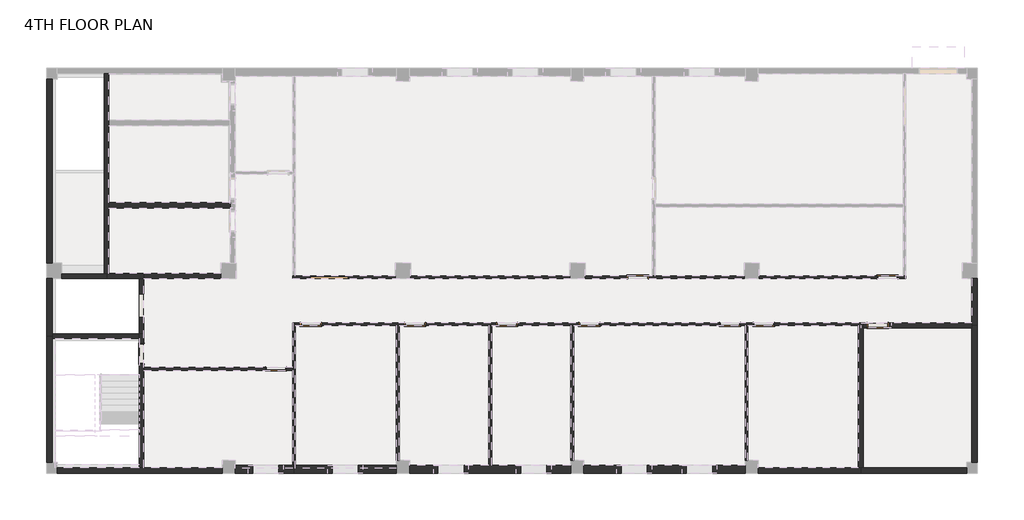
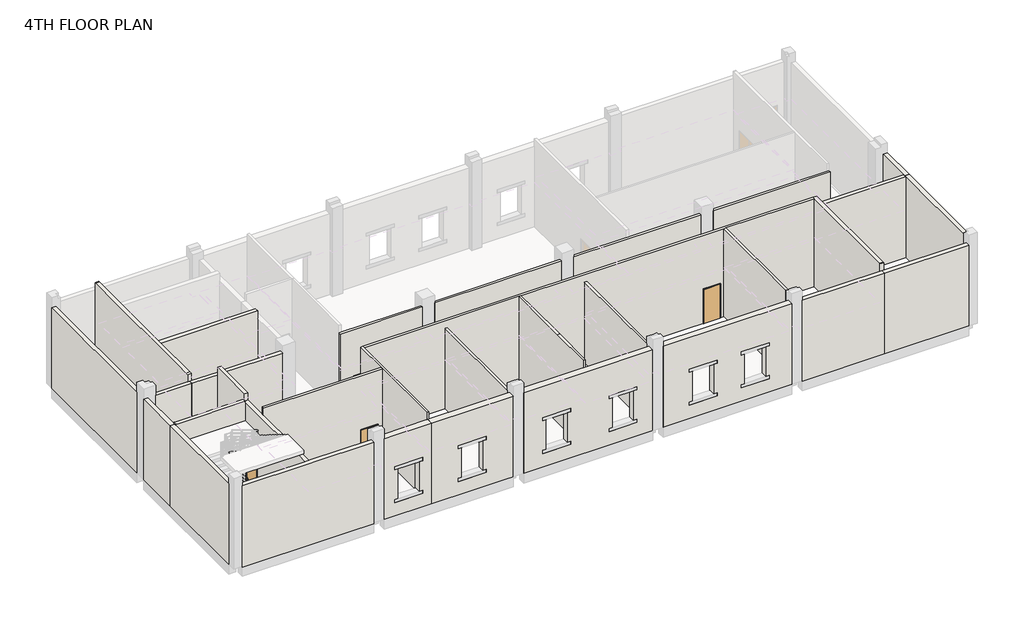
# One storey, part 1 of 6: 34 walls, 12 doors.
"""IFC4 building model written with IfcOpenShell, lengths in millimetres."""

import ifcopenshell
import ifcopenshell.guid

model = None  # the IFC model being written
_history = None  # IfcOwnerHistory: only IFC2X3 demands one
_inside = {}  # id of a spatial element -> (the spatial element, [elements in it])
_under = {}  # id of a project, library or spatial element -> (it, [spatial elements below it])
_declared = {}  # id of a project -> (the project, [libraries it declares])
_typed = {}  # id of a type object -> (the type object, [elements of that type])
_made_of = {}  # id of a material, layer set ... -> (it, [elements and type objects made of it])


def new_model(schema):
    """Start an empty IFC model of exactly this schema.

    Asked for "IFC4X3", IfcOpenShell would pick the latest addendum, in which some entities
    have other attributes; the version numbers below select the first issue.
    IFC2X3 requires an IfcOwnerHistory on every rooted entity: one is made here for all.
    """
    global model, _history
    if schema == "IFC4X3":
        model = ifcopenshell.file(schema_version=(4, 3, 0, 0))
    else:
        model = ifcopenshell.file(schema=schema)
    _inside.clear()
    _under.clear()
    _declared.clear()
    _typed.clear()
    _made_of.clear()
    _history = None
    if model.schema == "IFC2X3":
        org = make("IfcOrganization", Name="unknown")
        user = make(
            "IfcPersonAndOrganization",
            ThePerson=make("IfcPerson", FamilyName="unknown"),
            TheOrganization=org,
        )
        app = make(
            "IfcApplication",
            ApplicationDeveloper=org,
            Version="unknown",
            ApplicationFullName="unknown",
            ApplicationIdentifier="unknown",
        )
        _history = make(
            "IfcOwnerHistory",
            OwningUser=user,
            OwningApplication=app,
            ChangeAction="ADDED",
            CreationDate=0,
        )
    return model


def make(cls, **values):
    """One entity of the class cls with the attributes given. An attribute that is None is left unset."""
    return model.create_entity(
        cls, **{name: value for name, value in values.items() if value is not None}
    )


def rooted(cls, **values):
    """An entity with a GlobalId (a new one), such as an element, a storey or a relation."""
    return make(cls, GlobalId=ifcopenshell.guid.new(), OwnerHistory=_history, **values)


def si_unit(unit_type, name, prefix=None):
    """IfcSIUnit, for example si_unit("LENGTHUNIT", "METRE", prefix="MILLI")."""
    return make("IfcSIUnit", UnitType=unit_type, Prefix=prefix, Name=name)


def assignment(units):
    """IfcUnitAssignment: the units of a project."""
    return None if units is None else make("IfcUnitAssignment", Units=units)


def point(xyz):
    """IfcCartesianPoint."""
    return None if xyz is None else make("IfcCartesianPoint", Coordinates=xyz)


def direction(xyz):
    """IfcDirection."""
    return None if xyz is None else make("IfcDirection", DirectionRatios=xyz)


def frame(location, z_axis=None, x_axis=None):
    """IfcAxis2Placement3D, a coordinate frame: its origin and axes. An axis left out is left unset."""
    return make(
        "IfcAxis2Placement3D",
        Location=point(location),
        Axis=direction(z_axis),
        RefDirection=direction(x_axis),
    )


def origin():
    """The frame at (0, 0, 0) with its axes left unset."""
    return frame((0.0, 0.0, 0.0))


def origin_with_axes():
    """The frame at (0, 0, 0) with the z axis (0, 0, 1) and the x axis (1, 0, 0) written out."""
    return frame((0.0, 0.0, 0.0), z_axis=(0.0, 0.0, 1.0), x_axis=(1.0, 0.0, 0.0))


def place(relative_to, where):
    """IfcLocalPlacement: puts the frame where relative to a parent placement (None: the world)."""
    return make(
        "IfcLocalPlacement", PlacementRelTo=relative_to, RelativePlacement=where
    )


def context(
    kind, dimensions, precision=None, world=None, true_north=None, identifier=None
):
    """IfcGeometricRepresentationContext, for example the 3D "Model" context."""
    return make(
        "IfcGeometricRepresentationContext",
        ContextIdentifier=identifier,
        ContextType=kind,
        CoordinateSpaceDimension=dimensions,
        Precision=precision,
        WorldCoordinateSystem=world,
        TrueNorth=true_north,
    )


def project(units=None, contexts=None):
    """IfcProject with its units and contexts."""
    return rooted(
        "IfcProject",
        Name="project",
        RepresentationContexts=contexts,
        UnitsInContext=assignment(units),
    )


def spatial(cls, under=None, at=None, **own):
    """A site, building, storey or space (cls), placed at a placement, below another one or the project."""
    s = rooted(cls, ObjectPlacement=at, **own)
    if under is not None:
        _under.setdefault(under.id(), (under, []))[1].append(s)
    return s


def polyline(points):
    """IfcPolyline through the points."""
    return make("IfcPolyline", Points=[point(p) for p in points])


def outline(outer, holes=None, kind="AREA"):
    """IfcArbitraryClosedProfileDef: a profile drawn as a closed curve; with holes, ...WithVoids."""
    if holes is None:
        return make("IfcArbitraryClosedProfileDef", ProfileType=kind, OuterCurve=outer)
    return make(
        "IfcArbitraryProfileDefWithVoids",
        ProfileType=kind,
        OuterCurve=outer,
        InnerCurves=holes,
    )


def extrude(swept, where, along, depth):
    """IfcExtrudedAreaSolid: the profile swept, set in the frame where, extruded along a direction by depth."""
    return make(
        "IfcExtrudedAreaSolid",
        SweptArea=swept,
        Position=where,
        ExtrudedDirection=direction(along),
        Depth=depth,
    )


def faces_of(points, faces, orient=None, outer=None):
    """IfcFace entities. A face is a list of loops; a loop is a list of indices into points, from 0.

    orient and outer hold one flag for each loop. By default every Orientation is true, the
    first loop of a face is its IfcFaceOuterBound and the others are IfcFaceBound.
    """
    made = []
    for i, loops in enumerate(faces):
        bounds = []
        for j, loop in enumerate(loops):
            is_outer = j == 0 if outer is None else outer[i][j]
            bounds.append(
                make(
                    "IfcFaceOuterBound" if is_outer else "IfcFaceBound",
                    Bound=make("IfcPolyLoop", Polygon=[points[k] for k in loop]),
                    Orientation=True if orient is None else orient[i][j],
                )
            )
        made.append(make("IfcFace", Bounds=bounds))
    return made


def faceted_brep(points, faces, orient=None, outer=None, voids=None):
    """IfcFacetedBrep: a solid bounded by flat faces; with voids (closed shells), ...WithVoids."""
    shared = [point(p) for p in points]
    hull = make("IfcClosedShell", CfsFaces=faces_of(shared, faces, orient, outer))
    if voids is None:
        return make("IfcFacetedBrep", Outer=hull)
    return make(
        "IfcFacetedBrepWithVoids",
        Outer=hull,
        Voids=[
            make(cls, CfsFaces=faces_of(shared, fs, o, b)) for cls, fs, o, b in voids
        ],
    )


def shape(context_of_items, identifier, shape_type, items):
    """IfcShapeRepresentation: the items that make up one representation, for example the "Body"."""
    return make(
        "IfcShapeRepresentation",
        ContextOfItems=context_of_items,
        RepresentationIdentifier=identifier,
        RepresentationType=shape_type,
        Items=items,
    )


def source(mapping_origin, context_of_items, identifier, shape_type, items):
    """IfcRepresentationMap: a shape defined once, which mapped items show again and again."""
    return make(
        "IfcRepresentationMap",
        MappingOrigin=mapping_origin,
        MappedRepresentation=shape(context_of_items, identifier, shape_type, items),
    )


def transform(
    local_origin,
    x_axis=None,
    y_axis=None,
    z_axis=None,
    scale=None,
    scale2=None,
    scale3=None,
    uniform=True,
):
    """IfcCartesianTransformationOperator3D, or its non-uniform kind. x_axis, y_axis, z_axis: its Axis1, 2, 3."""
    if uniform:
        return make(
            "IfcCartesianTransformationOperator3D",
            Axis1=direction(x_axis),
            Axis2=direction(y_axis),
            LocalOrigin=point(local_origin),
            Scale=scale,
            Axis3=direction(z_axis),
        )
    return make(
        "IfcCartesianTransformationOperator3DnonUniform",
        Axis1=direction(x_axis),
        Axis2=direction(y_axis),
        LocalOrigin=point(local_origin),
        Scale=scale,
        Axis3=direction(z_axis),
        Scale2=scale2,
        Scale3=scale3,
    )


def mapped(mapping_source, mapping_target):
    """IfcMappedItem: shows the shape of a source again, moved by a transform."""
    return make(
        "IfcMappedItem", MappingSource=mapping_source, MappingTarget=mapping_target
    )


def made_of(thing, what):
    """Note that an element or type object is made of a material, layer set ...; save() writes the relation."""
    if what is not None:
        _made_of.setdefault(what.id(), (what, []))[1].append(thing)
    return thing


def element(
    cls,
    number,
    at=None,
    inside=None,
    cuts=None,
    type_object=None,
    material=None,
    context=None,
    identifier="Body",
    shape_type=None,
    held_by="IfcProductDefinitionShape",
    body=None,
    shapes=None,
    **own,
):
    """One element of the class cls, such as IfcWall. Its Tag is "e" and its number.

    at: its placement. inside: the storey or other place that contains it. cuts: it is an
    opening in that element (IfcRelVoidsElement). A single representation is given by context,
    identifier, shape_type and body (its items); several are given by shapes. held_by: the class
    of the entity that holds the representations. save() writes the other relations.
    """
    e = rooted(cls, Tag="e%d" % number, ObjectPlacement=at, **own)
    if body is not None:
        shapes = [shape(context, identifier, shape_type, body)]
    if shapes is not None:
        e.Representation = make(held_by, Representations=shapes)
    if inside is not None:
        _inside.setdefault(inside.id(), (inside, []))[1].append(e)
    if cuts is not None:
        rooted(
            "IfcRelVoidsElement", RelatingBuildingElement=cuts, RelatedOpeningElement=e
        )
    if type_object is not None:
        _typed.setdefault(type_object.id(), (type_object, []))[1].append(e)
    return made_of(e, material)


def aggregate(whole, parts):
    """IfcRelAggregates: a whole, such as a stair, and the parts it consists of."""
    return rooted("IfcRelAggregates", RelatingObject=whole, RelatedObjects=parts)


def save(model, path):
    """Write the relations noted so far, then the file.

    IfcRelAggregates (storeys below a building ...), IfcRelContainedInSpatialStructure (elements
    in a storey), IfcRelDefinesByType, IfcRelAssociatesMaterial and IfcRelDeclares: one each for
    every whole, place, type object, material and project.
    """
    for whole, parts in _under.values():
        aggregate(whole, parts)
    for where, things in _inside.values():
        rooted(
            "IfcRelContainedInSpatialStructure",
            RelatedElements=things,
            RelatingStructure=where,
        )
    for kind, things in _typed.values():
        rooted("IfcRelDefinesByType", RelatedObjects=things, RelatingType=kind)
    for what, things in _made_of.values():
        rooted("IfcRelAssociatesMaterial", RelatedObjects=things, RelatingMaterial=what)
    for by, libraries in _declared.values():
        rooted("IfcRelDeclares", RelatingContext=by, RelatedDefinitions=libraries)
    model.write(path)


def dr110_single_door_dr111_steel_door_1000x2100mm_481420e4(model_context):
    return source(origin(), model_context, "Body", "SolidModel", [
        extrude(outline(polyline([(470.0, -141.0), (-470.0, -141.0), (-470.0, -106.0), (470.0, -106.0), (470.0, -141.0)])), origin_with_axes(), (0.0, 0.0, 1.0), 2070.0),
        faceted_brep([(470.0, -141.0, 0.0), (470.0, -106.0, 0.0), (450.0, -106.0, 0.0), (450.0, 106.0, 0.0), (470.0, 106.0, 0.0), (470.0, 141.0, 0.0), (500.0, 141.0, 0.0), (500.0, -141.0, 0.0), (500.0, -141.0, 2100.0), (-500.0, -141.0, 2100.0), (-500.0, -141.0, 0.0), (-470.0, -141.0, 0.0), (-470.0, -141.0, 2070.0), (470.0, -141.0, 2070.0), (500.0, 141.0, 2100.0), (470.0, 141.0, 2070.0), (-470.0, 141.0, 2070.0), (-470.0, 141.0, 0.0), (-500.0, 141.0, 0.0), (-500.0, 141.0, 2100.0), (470.0, 106.0, 2070.0), (450.0, 106.0, 2050.0), (-450.0, 106.0, 2050.0), (-450.0, 106.0, 0.0), (-470.0, 106.0, 0.0), (-470.0, 106.0, 2070.0), (450.0, -106.0, 2050.0), (470.0, -106.0, 2070.0), (-470.0, -106.0, 2070.0), (-470.0, -106.0, 0.0), (-450.0, -106.0, 0.0), (-450.0, -106.0, 2050.0)], [[[0, 1, 2, 3, 4, 5, 6, 7]], [[7, 8, 9, 10, 11, 12, 13, 0]], [[6, 14, 8, 7]], [[5, 15, 16, 17, 18, 19, 14, 6]], [[4, 20, 15, 5]], [[3, 21, 22, 23, 24, 25, 20, 4]], [[2, 26, 21, 3]], [[1, 27, 28, 29, 30, 31, 26, 2]], [[0, 13, 27, 1]], [[12, 11, 29, 28]], [[11, 10, 18, 17, 24, 23, 30, 29]], [[19, 18, 10, 9]], [[25, 24, 17, 16]], [[31, 30, 23, 22]], [[14, 19, 9, 8]], [[20, 25, 16, 15]], [[26, 31, 22, 21]], [[13, 12, 28, 27]]]),
    ])


def dr110_single_door_dr111_steel_door_1000x2100mm_0699664c(model_context):
    return source(origin(), model_context, "Body", "SolidModel", [
        extrude(outline(polyline([(470.0, 92.5), (470.0, 57.5), (-470.0, 57.5), (-470.0, 92.5), (470.0, 92.5)])), origin_with_axes(), (0.0, 0.0, 1.0), 2070.0),
        faceted_brep([(470.0, 92.5, 0.0), (500.0, 92.5, 0.0), (500.0, -92.5, 0.0), (470.0, -92.5, 0.0), (470.0, -57.5, 0.0), (450.0, -57.5, 0.0), (450.0, 57.5, 0.0), (470.0, 57.5, 0.0), (470.0, 92.5, 2070.0), (-470.0, 92.5, 2070.0), (-470.0, 92.5, 0.0), (-500.0, 92.5, 0.0), (-500.0, 92.5, 2100.0), (500.0, 92.5, 2100.0), (500.0, -92.5, 2100.0), (-500.0, -92.5, 2100.0), (-500.0, -92.5, 0.0), (-470.0, -92.5, 0.0), (-470.0, -92.5, 2070.0), (470.0, -92.5, 2070.0), (470.0, -57.5, 2070.0), (-470.0, -57.5, 2070.0), (-470.0, -57.5, 0.0), (-450.0, -57.5, 0.0), (-450.0, -57.5, 2050.0), (450.0, -57.5, 2050.0), (450.0, 57.5, 2050.0), (-450.0, 57.5, 2050.0), (-450.0, 57.5, 0.0), (-470.0, 57.5, 0.0), (-470.0, 57.5, 2070.0), (470.0, 57.5, 2070.0)], [[[0, 1, 2, 3, 4, 5, 6, 7]], [[1, 0, 8, 9, 10, 11, 12, 13]], [[2, 1, 13, 14]], [[3, 2, 14, 15, 16, 17, 18, 19]], [[4, 3, 19, 20]], [[5, 4, 20, 21, 22, 23, 24, 25]], [[6, 5, 25, 26]], [[7, 6, 26, 27, 28, 29, 30, 31]], [[0, 7, 31, 8]], [[9, 30, 29, 10]], [[10, 29, 28, 23, 22, 17, 16, 11]], [[15, 12, 11, 16]], [[21, 18, 17, 22]], [[27, 24, 23, 28]], [[14, 13, 12, 15]], [[20, 19, 18, 21]], [[26, 25, 24, 27]], [[8, 31, 30, 9]]]),
    ])


def dr110_single_door_dr111_steel_door_1000x2100mm_67953bf6(model_context):
    return source(origin(), model_context, "Body", "SolidModel", [
        extrude(outline(polyline([(470.0, -92.5), (-470.0, -92.5), (-470.0, -57.5), (470.0, -57.5), (470.0, -92.5)])), origin_with_axes(), (0.0, 0.0, 1.0), 2070.0),
        faceted_brep([(470.0, -92.5, 0.0), (470.0, -57.5, 0.0), (450.0, -57.5, 0.0), (450.0, 57.5, 0.0), (470.0, 57.5, 0.0), (470.0, 92.5, 0.0), (500.0, 92.5, 0.0), (500.0, -92.5, 0.0), (500.0, -92.5, 2100.0), (-500.0, -92.5, 2100.0), (-500.0, -92.5, 0.0), (-470.0, -92.5, 0.0), (-470.0, -92.5, 2070.0), (470.0, -92.5, 2070.0), (500.0, 92.5, 2100.0), (470.0, 92.5, 2070.0), (-470.0, 92.5, 2070.0), (-470.0, 92.5, 0.0), (-500.0, 92.5, 0.0), (-500.0, 92.5, 2100.0), (470.0, 57.5, 2070.0), (450.0, 57.5, 2050.0), (-450.0, 57.5, 2050.0), (-450.0, 57.5, 0.0), (-470.0, 57.5, 0.0), (-470.0, 57.5, 2070.0), (450.0, -57.5, 2050.0), (470.0, -57.5, 2070.0), (-470.0, -57.5, 2070.0), (-470.0, -57.5, 0.0), (-450.0, -57.5, 0.0), (-450.0, -57.5, 2050.0)], [[[0, 1, 2, 3, 4, 5, 6, 7]], [[7, 8, 9, 10, 11, 12, 13, 0]], [[6, 14, 8, 7]], [[5, 15, 16, 17, 18, 19, 14, 6]], [[4, 20, 15, 5]], [[3, 21, 22, 23, 24, 25, 20, 4]], [[2, 26, 21, 3]], [[1, 27, 28, 29, 30, 31, 26, 2]], [[0, 13, 27, 1]], [[12, 11, 29, 28]], [[11, 10, 18, 17, 24, 23, 30, 29]], [[19, 18, 10, 9]], [[25, 24, 17, 16]], [[31, 30, 23, 22]], [[14, 19, 9, 8]], [[20, 25, 16, 15]], [[26, 31, 22, 21]], [[13, 12, 28, 27]]]),
    ])


def dr110_single_door_dr112_steel_door_1000x2100mm_panic_bar_81a01685(model_context):
    return source(origin(), model_context, "Body", "SolidModel", [
        extrude(outline(polyline([(470.0, -131.0), (-470.0, -131.0), (-470.0, -96.0), (470.0, -96.0), (470.0, -131.0)])), origin_with_axes(), (0.0, 0.0, 1.0), 2070.0),
        faceted_brep([(470.0, -131.0, 0.0), (470.0, -96.0, 0.0), (450.0, -96.0, 0.0), (450.0, 96.0, 0.0), (470.0, 96.0, 0.0), (470.0, 131.0, 0.0), (500.0, 131.0, 0.0), (500.0, -131.0, 0.0), (500.0, -131.0, 2100.0), (-500.0, -131.0, 2100.0), (-500.0, -131.0, 0.0), (-470.0, -131.0, 0.0), (-470.0, -131.0, 2070.0), (470.0, -131.0, 2070.0), (500.0, 131.0, 2100.0), (470.0, 131.0, 2070.0), (-470.0, 131.0, 2070.0), (-470.0, 131.0, 0.0), (-500.0, 131.0, 0.0), (-500.0, 131.0, 2100.0), (470.0, 96.0, 2070.0), (450.0, 96.0, 2050.0), (-450.0, 96.0, 2050.0), (-450.0, 96.0, 0.0), (-470.0, 96.0, 0.0), (-470.0, 96.0, 2070.0), (450.0, -96.0, 2050.0), (470.0, -96.0, 2070.0), (-470.0, -96.0, 2070.0), (-470.0, -96.0, 0.0), (-450.0, -96.0, 0.0), (-450.0, -96.0, 2050.0)], [[[0, 1, 2, 3, 4, 5, 6, 7]], [[7, 8, 9, 10, 11, 12, 13, 0]], [[6, 14, 8, 7]], [[5, 15, 16, 17, 18, 19, 14, 6]], [[4, 20, 15, 5]], [[3, 21, 22, 23, 24, 25, 20, 4]], [[2, 26, 21, 3]], [[1, 27, 28, 29, 30, 31, 26, 2]], [[0, 13, 27, 1]], [[12, 11, 29, 28]], [[11, 10, 18, 17, 24, 23, 30, 29]], [[19, 18, 10, 9]], [[25, 24, 17, 16]], [[31, 30, 23, 22]], [[14, 19, 9, 8]], [[20, 25, 16, 15]], [[26, 31, 22, 21]], [[13, 12, 28, 27]]]),
    ])


def dr120_double_door_dr121_steel_door_2000x2100mm_61964ec1(model_context):
    return source(origin(), model_context, "Body", "SolidModel", [
        extrude(outline(polyline([(880.0, 22.5), (0.0, 22.5), (0.0, 62.5), (880.0, 62.5), (880.0, 22.5)])), frame((0.0, 0.0, 20.0), z_axis=(0.0, 0.0, 1.0), x_axis=(1.0, 0.0, 0.0)), (0.0, 0.0, 1.0), 2060.0),
        extrude(outline(polyline([(0.0, 22.5), (-880.0, 22.5), (-880.0, 62.5), (0.0, 62.5), (0.0, 22.5)])), frame((0.0, 0.0, 20.0), z_axis=(0.0, 0.0, 1.0), x_axis=(1.0, 0.0, 0.0)), (0.0, 0.0, 1.0), 2060.0),
        faceted_brep([(900.0, -62.5, 2100.0), (900.0, 62.5, 2100.0), (-900.0, 62.5, 2100.0), (-900.0, -62.5, 2100.0), (865.0, 22.5, 2065.0), (865.0, -62.5, 2065.0), (-865.0, -62.5, 2065.0), (-865.0, 22.5, 2065.0), (880.0, 62.5, 2080.0), (880.0, 22.5, 2080.0), (-880.0, 22.5, 2080.0), (-880.0, 62.5, 2080.0), (-900.0, 62.5, 0.0), (-900.0, -62.5, 0.0), (-865.0, -62.5, 35.0), (-865.0, 22.5, 35.0), (-880.0, 22.5, 20.0), (-880.0, 62.5, 20.0), (900.0, 62.5, 0.0), (880.0, 62.5, 20.0), (900.0, -62.5, 0.0), (865.0, -62.5, 35.0), (865.0, 22.5, 35.0), (880.0, 22.5, 20.0)], [[[0, 1, 2, 3]], [[4, 5, 6, 7]], [[8, 9, 10, 11]], [[3, 2, 12, 13]], [[7, 6, 14, 15]], [[11, 10, 16, 17]], [[18, 12, 2, 1], [8, 11, 17, 19]], [[13, 12, 18, 20]], [[0, 3, 13, 20], [21, 14, 6, 5]], [[15, 14, 21, 22]], [[23, 16, 10, 9], [4, 7, 15, 22]], [[17, 16, 23, 19]], [[20, 18, 1, 0]], [[22, 21, 5, 4]], [[19, 23, 9, 8]]]),
    ])


model = new_model("IFC4")

# Units and contexts
model_context = context("Model", 3, world=origin())
ifc_project = project(units=[si_unit("LENGTHUNIT", "METRE", prefix="MILLI")], contexts=[model_context])

# Site, building, storey
site = spatial("IfcSite", under=ifc_project)
building = spatial("IfcBuilding", under=site)
storey = spatial("IfcBuildingStorey", under=building, Name="4TH FLOOR PLAN", Elevation=16100.005241)

# Doors
placement = place(None, origin())
dr110_single_door_dr111_steel_door_1000x2100mm_shape = dr110_single_door_dr111_steel_door_1000x2100mm_481420e4(model_context)
element("IfcDoor", 1, ObjectType="DR110-Single Door : DR111-Steel Door-1000x2100mm", at=placement, inside=storey, context=model_context, shape_type="MappedRepresentation", body=[
    mapped(dr110_single_door_dr111_steel_door_1000x2100mm_shape, transform((37775.0, 27499.5208589, 16100.005241), x_axis=(1.0, 0.0, 0.0), y_axis=(0.0, 1.0, 0.0), z_axis=(0.0, 0.0, 1.0))),
])
dr110_single_door_dr111_steel_door_1000x2100mm_2_shape = dr110_single_door_dr111_steel_door_1000x2100mm_0699664c(model_context)
element("IfcDoor", 2, ObjectType="DR110-Single Door : DR111-Steel Door-1000x2100mm", at=placement, inside=storey, context=model_context, shape_type="MappedRepresentation", body=[
    mapped(dr110_single_door_dr111_steel_door_1000x2100mm_2_shape, transform((10170.0, 25499.5208589, 16100.005241), x_axis=(-1.0, 0.0, 0.0), y_axis=(0.0, -1.0, 0.0), z_axis=(0.0, 0.0, 1.0))),
])
element("IfcDoor", 3, ObjectType="DR110-Single Door : DR111-Steel Door-1000x2100mm", at=placement, inside=storey, context=model_context, shape_type="MappedRepresentation", body=[
    mapped(dr110_single_door_dr111_steel_door_1000x2100mm_2_shape, transform((31000.0, 27547.0208589, 16100.005241), x_axis=(-1.0, 0.0, 0.0), y_axis=(0.0, -1.0, 0.0), z_axis=(0.0, 0.0, 1.0))),
])
dr110_single_door_dr111_steel_door_1000x2100mm_3_shape = dr110_single_door_dr111_steel_door_1000x2100mm_67953bf6(model_context)
element("IfcDoor", 4, ObjectType="DR110-Single Door : DR111-Steel Door-1000x2100mm", at=placement, inside=storey, context=model_context, shape_type="MappedRepresentation", body=[
    mapped(dr110_single_door_dr111_steel_door_1000x2100mm_3_shape, transform((38225.0, 29712.0208589, 16100.005241), x_axis=(-1.0, 0.0, 0.0), y_axis=(0.0, -1.0, 0.0), z_axis=(0.0, 0.0, 1.0))),
])
element("IfcDoor", 5, ObjectType="DR110-Single Door : DR111-Steel Door-1000x2100mm", at=placement, inside=storey, context=model_context, shape_type="MappedRepresentation", body=[
    mapped(dr110_single_door_dr111_steel_door_1000x2100mm_3_shape, transform((26770.0, 29712.0208589, 16100.005241), x_axis=(-1.0, 0.0, 0.0), y_axis=(0.0, -1.0, 0.0), z_axis=(0.0, 0.0, 1.0))),
])
element("IfcDoor", 6, ObjectType="DR110-Single Door : DR111-Steel Door-1000x2100mm", at=placement, inside=storey, context=model_context, shape_type="MappedRepresentation", body=[
    mapped(dr110_single_door_dr111_steel_door_1000x2100mm_3_shape, transform((11775.0, 27547.0208589, 16100.005241), x_axis=(1.0, 0.0, 0.0), y_axis=(0.0, 1.0, 0.0), z_axis=(0.0, 0.0, 1.0))),
])
element("IfcDoor", 7, ObjectType="DR110-Single Door : DR111-Steel Door-1000x2100mm", at=placement, inside=storey, context=model_context, shape_type="MappedRepresentation", body=[
    mapped(dr110_single_door_dr111_steel_door_1000x2100mm_3_shape, transform((16550.0, 27547.0208589, 16100.005241), x_axis=(1.0, 0.0, 0.0), y_axis=(0.0, 1.0, 0.0), z_axis=(0.0, 0.0, 1.0))),
])
element("IfcDoor", 8, ObjectType="DR110-Single Door : DR111-Steel Door-1000x2100mm", at=placement, inside=storey, context=model_context, shape_type="MappedRepresentation", body=[
    mapped(dr110_single_door_dr111_steel_door_1000x2100mm_3_shape, transform((20775.0, 27547.0208589, 16100.005241), x_axis=(1.0, 0.0, 0.0), y_axis=(0.0, 1.0, 0.0), z_axis=(0.0, 0.0, 1.0))),
])
element("IfcDoor", 9, ObjectType="DR110-Single Door : DR111-Steel Door-1000x2100mm", at=placement, inside=storey, context=model_context, shape_type="MappedRepresentation", body=[
    mapped(dr110_single_door_dr111_steel_door_1000x2100mm_3_shape, transform((24550.0, 27547.0208589, 16100.005241), x_axis=(1.0, 0.0, 0.0), y_axis=(0.0, 1.0, 0.0), z_axis=(0.0, 0.0, 1.0))),
])
element("IfcDoor", 10, ObjectType="DR110-Single Door : DR111-Steel Door-1000x2100mm", at=placement, inside=storey, context=model_context, shape_type="MappedRepresentation", body=[
    mapped(dr110_single_door_dr111_steel_door_1000x2100mm_3_shape, transform((32550.0, 27547.0208589, 16100.005241), x_axis=(1.0, 0.0, 0.0), y_axis=(0.0, 1.0, 0.0), z_axis=(0.0, 0.0, 1.0))),
])
dr110_single_door_dr112_steel_door_1000x2100mm_panic_bar_shape = dr110_single_door_dr112_steel_door_1000x2100mm_panic_bar_81a01685(model_context)
element("IfcDoor", 11, ObjectType="DR110-Single Door : DR112-Steel Door-1000x2100mm_Panic Bar", at=placement, inside=storey, context=model_context, shape_type="MappedRepresentation", body=[
    mapped(dr110_single_door_dr112_steel_door_1000x2100mm_panic_bar_shape, transform((4000.0, 26199.5208589, 16100.005241), x_axis=(0.0, -1.0, 0.0), y_axis=(1.0, 0.0, 0.0), z_axis=(0.0, 0.0, 1.0))),
])
dr120_double_door_dr121_steel_door_2000x2100mm_shape = dr120_double_door_dr121_steel_door_2000x2100mm_61964ec1(model_context)
element("IfcDoor", 12, ObjectType="DR120-Double Door : DR121-Steel Door-2000x2100mm", at=placement, inside=storey, context=model_context, shape_type="MappedRepresentation", body=[
    mapped(dr120_double_door_dr121_steel_door_2000x2100mm_shape, transform((12620.0, 29712.0208589, 16100.005241), x_axis=(1.0, 0.0, 0.0), y_axis=(0.0, 1.0, 0.0), z_axis=(0.0, 0.0, 1.0))),
])

# Walls
element("IfcWall", 13, at=placement, inside=storey, context=model_context, shape_type="Brep", body=[
    faceted_brep([(-351.0, 38799.5208589, 16100.005241), (-351.0, 30349.5208589, 16100.005241), (-351.0, 30349.5208589, 21000.005241), (-351.0, 38799.5208589, 21000.005241), (-100.0, 38799.5208589, 16100.005241), (-100.0, 38799.5208589, 21000.005241), (-100.0, 30349.5208589, 21000.005241), (-100.0, 30349.5208589, 16100.005241), (-350.0, 38799.5208589, 16100.005241), (-350.0, 30349.5208589, 16100.005241), (-350.0, 30349.5208589, 21000.005241), (-350.0, 38799.5208589, 21000.005241)], [[[0, 1, 2, 3]], [[4, 5, 6, 7]], [[1, 0, 8, 4, 7, 9]], [[2, 1, 9, 7, 6, 10]], [[3, 2, 10, 6, 5, 11]], [[0, 3, 11, 5, 4, 8]]]),
])
element("IfcWall", 14, at=placement, inside=storey, context=model_context, shape_type="Brep", body=[
    faceted_brep([(42099.0, 27499.5208589, 16100.005241), (42099.0, 21199.5208589, 16100.005241), (42099.0, 21199.5208589, 21000.005241), (42099.0, 27499.5208589, 21000.005241), (42351.0, 27499.5208589, 16100.005241), (42351.0, 27499.5208589, 21000.005241), (42351.0, 21199.5208589, 21000.005241), (42351.0, 21199.5208589, 16100.005241), (42350.0, 21199.5208589, 16100.005241), (42350.0, 21199.5208589, 21000.005241)], [[[0, 1, 2, 3]], [[4, 5, 6, 7]], [[1, 0, 4, 7, 8]], [[2, 1, 8, 7, 6, 9]], [[3, 2, 9, 6, 5]], [[0, 3, 5, 4]]]),
])
element("IfcWall", 15, at=placement, inside=storey, context=model_context, shape_type="Brep", body=[
    faceted_brep([(37000.0, 20950.5208589, 16100.005241), (32300.0, 20950.5208589, 16100.005241), (32300.0, 20950.5208589, 21000.005241), (37000.0, 20950.5208589, 21000.005241), (37000.0, 20698.5208589, 16100.005241), (37000.0, 20698.5208589, 21000.005241), (32300.0, 20698.5208589, 21000.005241), (32300.0, 20698.5208589, 16100.005241), (32300.0, 20699.5208589, 16100.005241), (32300.0, 20699.5208589, 21000.005241)], [[[0, 1, 2, 3]], [[4, 5, 6, 7]], [[1, 0, 4, 7, 8]], [[2, 1, 8, 7, 6, 9]], [[3, 2, 9, 6, 5]], [[0, 3, 5, 4]]]),
])
element("IfcWall", 16, at=placement, inside=storey, context=model_context, shape_type="Brep", body=[
    faceted_brep([(2400.0, 29649.5208589, 16050.005241), (3900.0, 29649.5208589, 16050.005241), (4000.0, 29649.5208589, 16050.005241), (4101.0, 29649.5208589, 16050.005241), (4101.0, 29649.5208589, 21000.005241), (2400.0, 29649.5208589, 21000.005241), (2400.0, 29849.5208589, 16050.005241), (2400.0, 29849.5208589, 21000.005241), (4101.0, 29849.5208589, 21000.005241), (4101.0, 29849.5208589, 16050.005241), (4000.0, 29849.5208589, 16050.005241)], [[[0, 1, 2, 3, 4, 5]], [[6, 7, 8, 9, 10]], [[3, 2, 1, 0, 6, 10, 9]], [[5, 4, 8, 7]], [[0, 5, 7, 6]], [[4, 3, 9, 8]]]),
])
element("IfcWall", 17, at=placement, inside=storey, context=model_context, shape_type="Brep", body=[
    faceted_brep([(2510.0, 29849.5208589, 16050.005241), (2510.0, 32874.5208589, 16050.005241), (2510.0, 33124.5208589, 16050.005241), (2510.0, 36674.5208589, 16050.005241), (2510.0, 36924.5208589, 16050.005241), (2510.0, 39049.5208589, 16050.005241), (2510.0, 39049.5208589, 16100.005241), (2510.0, 39049.5208589, 19100.005241), (2510.0, 39049.5208589, 21450.005241), (2510.0, 38999.7368538, 21450.005241), (2510.0, 36924.5208589, 21450.005241), (2510.0, 36674.5208589, 21450.005241), (2510.0, 33124.5208589, 21450.005241), (2510.0, 32874.5208589, 21450.005241), (2510.0, 29999.5208589, 21450.005241), (2510.0, 29849.5208589, 21450.005241), (2290.0, 29849.5208589, 16050.005241), (2290.0, 29849.5208589, 21450.005241), (2290.0, 29999.5208589, 21450.005241), (2290.0, 38999.7368538, 21450.005241), (2290.0, 39049.5208589, 21450.005241), (2290.0, 39049.5208589, 16050.005241)], [[[0, 1, 2, 3, 4, 5, 6, 7, 8, 9, 10, 11, 12, 13, 14, 15]], [[16, 17, 18, 19, 20, 21]], [[5, 4, 3, 2, 1, 0, 16, 21]], [[8, 7, 6, 5, 21, 20]], [[0, 15, 17, 16]], [[9, 8, 20, 19]], [[15, 14, 18, 17]], [[14, 13, 12, 11, 10, 9, 19, 18]]]),
])
element("IfcWall", 18, at=placement, inside=storey, context=model_context, shape_type="Brep", body=[
    faceted_brep([(36889.0, 27610.5208589, 16050.005241), (36889.0, 20949.5208589, 16050.005241), (36889.0, 20949.5208589, 21450.005241), (36889.0, 20999.5208589, 21450.005241), (36889.0, 27610.5208589, 21450.005241), (37111.0, 20949.5208589, 16050.005241), (37111.0, 27388.5208589, 16050.005241), (37111.0, 27610.5208589, 16050.005241), (37111.0, 27610.5208589, 18200.005241), (37111.0, 27388.5208589, 18200.005241), (37111.0, 27388.5208589, 18390.005241), (37111.0, 27610.5208589, 18390.005241), (37111.0, 27610.5208589, 21000.005241), (37111.0, 27610.5208589, 21450.005241), (37111.0, 20999.5208589, 21450.005241), (37111.0, 20949.5208589, 21450.005241), (37030.0, 27610.5208589, 18390.005241), (37030.0, 27610.5208589, 18200.005241), (37030.0, 27388.5208589, 18200.005241), (37030.0, 27388.5208589, 18390.005241)], [[[0, 1, 2, 3, 4]], [[5, 6, 7, 8, 9, 10, 11, 12, 13, 14, 15]], [[1, 0, 7, 6, 5]], [[2, 1, 5, 15]], [[0, 4, 13, 12, 11, 16, 17, 8, 7]], [[18, 19, 10, 9]], [[19, 16, 11, 10]], [[19, 18, 17, 16]], [[17, 18, 9, 8]], [[2, 15, 14, 3]], [[13, 4, 3, 14]]]),
])
element("IfcWall", 19, at=placement, inside=storey, context=model_context, shape_type="SweptSolid", body=[
    extrude(outline(polyline([(16050.005241, 37111.0), (16050.005241, 42099.0), (21000.005241, 42099.0), (21000.005241, 37111.0), (18390.005241, 37111.0), (18390.005241, 38400.0), (18200.005241, 38400.0), (18200.005241, 38275.0), (16100.005241, 38275.0), (16100.005241, 37275.0), (18200.005241, 37275.0), (18200.005241, 37111.0), (16050.005241, 37111.0)])), frame((0.0, 27388.5208589, 0.0), z_axis=(0.0, 1.0, 0.0), x_axis=(0.0, 0.0, 1.0)), (0.0, 0.0, 1.0), 222.0),
])
element("IfcWall", 20, at=placement, inside=storey, context=model_context, shape_type="SweptSolid", body=[
    extrude(outline(polyline([(8064.5, 32874.5208589), (2510.0, 32874.5208589), (2510.0, 33124.5208589), (8064.5, 33124.5208589), (8064.5, 32874.5208589)])), frame((0.0, 0.0, 16050.005241), z_axis=(0.0, 0.0, 1.0), x_axis=(1.0, 0.0, 0.0)), (0.0, 0.0, 1.0), 5400.0),
])
element("IfcWall", 21, at=placement, inside=storey, context=model_context, shape_type="SweptSolid", body=[
    extrude(outline(polyline([(4100.0, 29887.5208589), (7650.0, 29887.5208589), (7650.0, 29651.5208589), (4100.0, 29651.5208589), (4100.0, 29887.5208589)])), frame((0.0, 0.0, 16100.005241), z_axis=(0.0, 0.0, 1.0), x_axis=(1.0, 0.0, 0.0)), (0.0, 0.0, 1.0), 4900.0),
])
element("IfcWall", 22, at=placement, inside=storey, context=model_context, shape_type="Brep", body=[
    faceted_brep([(150.0, 20698.5208589, 16050.005241), (7700.0, 20698.5208589, 16050.005241), (7700.0, 20698.5208589, 21000.005241), (150.0, 20698.5208589, 21000.005241), (150.0, 20950.5208589, 16050.005241), (150.0, 20950.5208589, 16100.005241), (150.0, 20950.5208589, 21000.005241), (3899.0, 20950.5208589, 21000.005241), (4101.0, 20950.5208589, 21000.005241), (7700.0, 20950.5208589, 21000.005241), (7700.0, 20950.5208589, 16100.005241), (7700.0, 20950.5208589, 16050.005241), (4101.0, 20950.5208589, 16050.005241), (3899.0, 20950.5208589, 16050.005241), (150.0, 20699.5208589, 16050.005241), (7700.0, 20699.5208589, 16050.005241), (7700.0, 20699.5208589, 21000.005241), (150.0, 20699.5208589, 21000.005241)], [[[0, 1, 2, 3]], [[4, 5, 6, 7, 8, 9, 10, 11, 12, 13]], [[1, 0, 14, 4, 13, 12, 11, 15]], [[2, 1, 15, 11, 10, 9, 16]], [[3, 2, 16, 9, 8, 7, 6, 17]], [[0, 3, 17, 6, 5, 4, 14]]]),
])
element("IfcWall", 23, at=placement, inside=storey, context=model_context, shape_type="Brep", body=[
    faceted_brep([(-351.0, 26999.5208589, 16100.005241), (-351.0, 21199.5208589, 16100.005241), (-351.0, 21199.5208589, 21000.005241), (-351.0, 26999.5208589, 21000.005241), (-99.0, 26999.5208589, 16100.005241), (-99.0, 26999.5208589, 21000.005241), (-99.0, 26899.0208589, 21000.005241), (-99.0, 21199.5208589, 21000.005241), (-99.0, 21199.5208589, 16100.005241), (-99.0, 26899.0208589, 16100.005241), (-100.0, 26999.5208589, 16100.005241), (-350.0, 21199.5208589, 16100.005241), (-350.0, 21199.5208589, 21000.005241), (-100.0, 26999.5208589, 21000.005241)], [[[0, 1, 2, 3]], [[4, 5, 6, 7, 8, 9]], [[1, 0, 10, 4, 9, 8, 11]], [[2, 1, 11, 8, 7, 12]], [[3, 2, 12, 7, 6, 5, 13]], [[0, 3, 13, 5, 4, 10]]]),
])
element("IfcWall", 24, at=placement, inside=storey, context=model_context, shape_type="Brep", body=[
    faceted_brep([(4101.0, 20950.5208589, 16050.005241), (4101.0, 20999.5208589, 16050.005241), (4101.0, 27100.0208589, 16050.005241), (4101.0, 27100.0208589, 21000.005241), (4101.0, 26999.5208589, 21000.005241), (4101.0, 20950.5208589, 21000.005241), (4101.0, 20950.5208589, 16100.005241), (4101.0, 25699.5208589, 16100.005241), (4101.0, 25699.5208589, 18200.005241), (4101.0, 26699.5208589, 18200.005241), (4101.0, 26699.5208589, 16100.005241), (3899.0, 27100.0208589, 16050.005241), (3899.0, 26899.0208589, 16050.005241), (3899.0, 21099.5208589, 16050.005241), (3899.0, 20950.5208589, 16050.005241), (3899.0, 20950.5208589, 16100.005241), (3899.0, 20950.5208589, 21000.005241), (3899.0, 27100.0208589, 21000.005241), (3899.0, 25699.5208589, 18200.005241), (3899.0, 25699.5208589, 16100.005241), (3899.0, 26699.5208589, 16100.005241), (3899.0, 26699.5208589, 18200.005241), (3900.0, 27100.0208589, 16050.005241), (3900.0, 27100.0208589, 21000.005241)], [[[0, 1, 2, 3, 4, 5, 6], [7, 8, 9, 10]], [[11, 12, 13, 14, 15, 16, 17], [18, 19, 20, 21]], [[2, 1, 0, 14, 13, 12, 11, 22]], [[5, 4, 3, 23, 17, 16]], [[7, 19, 18, 8]], [[8, 18, 21, 9]], [[9, 21, 20, 10]], [[19, 7, 10, 20]], [[3, 2, 22, 11, 17, 23]], [[0, 6, 5, 16, 15, 14]]]),
])
element("IfcWall", 25, at=placement, inside=storey, context=model_context, shape_type="Brep", body=[
    faceted_brep([(-99.0, 26899.0208589, 16050.005241), (50.0, 26899.0208589, 16050.005241), (3899.0, 26899.0208589, 16050.005241), (3899.0, 26899.0208589, 16100.005241), (3899.0, 26899.0208589, 21050.005241), (50.0, 26899.0208589, 21050.005241), (-99.0, 26899.0208589, 21050.005241), (-99.0, 26899.0208589, 21000.005241), (-99.0, 26899.0208589, 16100.005241), (-100.0, 27100.0208589, 16050.005241), (-100.0, 27100.0208589, 16100.005241), (-100.0, 27100.0208589, 21000.005241), (-100.0, 27100.0208589, 21050.005241), (50.0, 27100.0208589, 21050.005241), (3899.0, 27100.0208589, 21050.005241), (3899.0, 27100.0208589, 21000.005241), (3899.0, 27100.0208589, 16050.005241), (50.0, 27100.0208589, 16050.005241), (-99.0, 26999.5208589, 16050.005241), (-100.0, 26999.5208589, 16050.005241), (-100.0, 26999.5208589, 21050.005241), (-99.0, 26999.5208589, 21050.005241), (-99.0, 26999.5208589, 21000.005241), (-99.0, 26999.5208589, 16100.005241), (-100.0, 26999.5208589, 21000.005241), (-100.0, 26999.5208589, 16100.005241)], [[[0, 1, 2, 3, 4, 5, 6, 7, 8]], [[9, 10, 11, 12, 13, 14, 15, 16, 17]], [[2, 1, 0, 18, 19, 9, 17, 16]], [[6, 5, 4, 14, 13, 12, 20, 21]], [[4, 3, 2, 16, 15, 14]], [[0, 8, 7, 6, 21, 22, 23, 18]], [[21, 20, 24, 25, 19, 18, 23, 22]], [[20, 12, 11, 10, 9, 19, 25, 24]]]),
])
element("IfcWall", 26, at=placement, inside=storey, context=model_context, shape_type="Brep", body=[
    faceted_brep([(4101.0, 29649.5208589, 21450.005241), (4101.0, 26999.5208589, 21450.005241), (4101.0, 26999.5208589, 21000.005241), (4101.0, 27100.0208589, 21000.005241), (4101.0, 27100.0208589, 16050.005241), (4101.0, 29649.5208589, 16050.005241), (4101.0, 29649.5208589, 21000.005241), (4101.0, 28929.5208589, 16100.005241), (4101.0, 27849.5208589, 16100.005241), (4101.0, 27849.5208589, 18300.005241), (4101.0, 28929.5208589, 18300.005241), (3900.0, 26999.5208589, 21450.005241), (3900.0, 29649.5208589, 21450.005241), (3900.0, 29649.5208589, 16050.005241), (3900.0, 27100.0208589, 16050.005241), (3900.0, 27100.0208589, 21000.005241), (3900.0, 26999.5208589, 21000.005241), (3900.0, 27849.5208589, 16100.005241), (3900.0, 28929.5208589, 16100.005241), (3900.0, 28929.5208589, 18300.005241), (3900.0, 27849.5208589, 18300.005241), (4000.0, 29649.5208589, 16050.005241), (4000.0, 29649.5208589, 21450.005241), (4000.0, 26999.5208589, 21450.005241)], [[[0, 1, 2, 3, 4, 5, 6], [7, 8, 9, 10]], [[11, 12, 13, 14, 15, 16], [17, 18, 19, 20]], [[13, 21, 5, 4, 14]], [[1, 0, 22, 12, 11, 23]], [[1, 23, 11, 16, 2]], [[7, 18, 17, 8]], [[8, 17, 20, 9]], [[18, 7, 10, 19]], [[9, 20, 19, 10]], [[12, 22, 0, 6, 5, 21, 13]], [[15, 3, 2, 16]], [[3, 15, 14, 4]]]),
])
element("IfcWall", 27, at=placement, inside=storey, context=model_context, shape_type="Brep", body=[
    faceted_brep([(350.0, 29649.5208589, 21000.005241), (350.0, 29649.5208589, 16100.005241), (350.0, 29649.5208589, 16050.005241), (2400.0, 29649.5208589, 16050.005241), (2400.0, 29649.5208589, 21000.005241), (350.0, 29849.5208589, 16050.005241), (350.0, 29849.5208589, 16100.005241), (350.0, 29849.5208589, 21000.005241), (2400.0, 29849.5208589, 21000.005241), (2400.0, 29849.5208589, 16050.005241)], [[[0, 1, 2, 3, 4]], [[5, 6, 7, 8, 9]], [[2, 5, 9, 3]], [[7, 0, 4, 8]], [[2, 1, 0, 7, 6, 5]], [[4, 3, 9, 8]]]),
])
element("IfcWall", 28, at=placement, inside=storey, context=model_context, shape_type="Brep", body=[
    faceted_brep([(42099.0, 29649.5208589, 16100.005241), (42099.0, 27499.5208589, 16100.005241), (42099.0, 27499.5208589, 21000.005241), (42099.0, 29649.5208589, 21000.005241), (42351.0, 29649.5208589, 16100.005241), (42351.0, 29649.5208589, 21000.005241), (42351.0, 27499.5208589, 21000.005241), (42351.0, 27499.5208589, 16100.005241), (42350.0, 29649.5208589, 16100.005241), (42350.0, 29649.5208589, 21000.005241)], [[[0, 1, 2, 3]], [[4, 5, 6, 7]], [[1, 0, 8, 4, 7]], [[2, 1, 7, 6]], [[3, 2, 6, 5, 9]], [[0, 3, 9, 5, 4, 8]]]),
])
element("IfcWall", 29, at=placement, inside=storey, context=model_context, shape_type="Brep", body=[
    faceted_brep([(41850.0, 20950.5208589, 16100.005241), (37000.0, 20950.5208589, 16100.005241), (37000.0, 20950.5208589, 21000.005241), (41850.0, 20950.5208589, 21000.005241), (41850.0, 20698.5208589, 16100.005241), (41850.0, 20698.5208589, 21000.005241), (37000.0, 20698.5208589, 21000.005241), (37000.0, 20698.5208589, 16100.005241), (41850.0, 20699.5208589, 16100.005241), (41850.0, 20699.5208589, 21000.005241)], [[[0, 1, 2, 3]], [[4, 5, 6, 7]], [[1, 0, 8, 4, 7]], [[2, 1, 7, 6]], [[3, 2, 6, 5, 9]], [[0, 3, 9, 5, 4, 8]]]),
])
element("IfcWall", 30, at=placement, inside=storey, context=model_context, shape_type="SweptSolid", body=[
    extrude(outline(polyline([(2510.0, 29887.0208589), (4100.0, 29887.0208589), (4100.0, 29857.0208589), (2510.0, 29857.0208589), (2510.0, 29887.0208589)])), frame((0.0, 0.0, 16100.005241), z_axis=(0.0, 0.0, 1.0), x_axis=(1.0, 0.0, 0.0)), (0.0, 0.0, 1.0), 3000.0),
])
element("IfcWall", 31, at=placement, inside=storey, context=model_context, shape_type="Brep", body=[
    faceted_brep([(-351.0, 29649.5208589, 16100.005241), (-351.0, 26999.5208589, 16100.005241), (-351.0, 26999.5208589, 21000.005241), (-351.0, 29649.5208589, 21000.005241), (-100.0, 29649.5208589, 16100.005241), (-100.0, 29649.5208589, 21000.005241), (-100.0, 27100.0208589, 21000.005241), (-100.0, 26999.5208589, 21000.005241), (-100.0, 26999.5208589, 16100.005241), (-100.0, 27100.0208589, 16100.005241), (-350.0, 29649.5208589, 16100.005241), (-350.0, 29649.5208589, 21000.005241)], [[[0, 1, 2, 3]], [[4, 5, 6, 7, 8, 9]], [[1, 0, 10, 4, 9, 8]], [[2, 1, 8, 7]], [[3, 2, 7, 6, 5, 11]], [[0, 3, 11, 5, 4, 10]]]),
])
element("IfcWall", 32, ObjectType="WA452_Int. Gypsum Wall 2 Layer_2 Hr_125", at=placement, inside=storey, context=model_context, shape_type="Brep", body=[
    faceted_brep([(10937.5, 29774.5208589, 21000.005241), (15650.0, 29774.5208589, 21000.005241), (15650.0, 29774.5208589, 16100.005241), (13520.0, 29774.5208589, 16100.005241), (13520.0, 29774.5208589, 18200.005241), (11720.0, 29774.5208589, 18200.005241), (11720.0, 29774.5208589, 16100.005241), (11062.5, 29774.5208589, 16100.005241), (10937.5, 29774.5208589, 16100.005241), (15650.0, 29649.5208589, 21000.005241), (10937.5, 29649.5208589, 21000.005241), (10937.5, 29649.5208589, 16100.005241), (11720.0, 29649.5208589, 16100.005241), (11720.0, 29649.5208589, 18200.005241), (13520.0, 29649.5208589, 18200.005241), (13520.0, 29649.5208589, 16100.005241), (15650.0, 29649.5208589, 16100.005241)], [[[0, 1, 2, 3, 4, 5, 6, 7, 8]], [[9, 10, 11, 12, 13, 14, 15, 16]], [[2, 16, 15, 3]], [[11, 8, 7, 6, 12]], [[1, 0, 10, 9]], [[2, 1, 9, 16]], [[14, 4, 3, 15]], [[4, 14, 13, 5]], [[5, 13, 12, 6]], [[0, 8, 11, 10]]]),
])
element("IfcWall", 33, ObjectType="WA452_Int. Gypsum Wall 2 Layer_2 Hr_125", at=placement, inside=storey, context=model_context, shape_type="SweptSolid", body=[
    extrude(outline(polyline([(21450.005241, 4100.0), (16100.005241, 4100.0), (16100.005241, 9670.0), (18200.005241, 9670.0), (18200.005241, 10670.0), (16100.005241, 10670.0), (16100.005241, 10937.5), (21450.005241, 10937.5), (21450.005241, 4100.0)])), frame((0.0, 25437.0208589, 0.0), z_axis=(0.0, 1.0, 0.0), x_axis=(0.0, 0.0, 1.0)), (0.0, 0.0, 1.0), 125.0),
])
element("IfcWall", 34, ObjectType="WA452_Int. Gypsum Wall 2 Layer_2 Hr_125", at=placement, inside=storey, context=model_context, shape_type="SweptSolid", body=[
    extrude(outline(polyline([(27484.5208589, 16100.005241), (21084.5208589, 16100.005241), (21084.5208589, 21450.005241), (23649.5208589, 21450.005241), (26349.5208589, 21450.005241), (27484.5208589, 21450.005241), (27484.5208589, 16100.005241)])), frame((19937.5, 0.0, 0.0), z_axis=(1.0, 0.0, 0.0), x_axis=(0.0, 1.0, 0.0)), (0.0, 0.0, 1.0), 125.0),
])
element("IfcWall", 35, ObjectType="WA452_Int. Gypsum Wall 2 Layer_2 Hr_125", at=placement, inside=storey, context=model_context, shape_type="SweptSolid", body=[
    extrude(outline(polyline([(31700.0, 21299.5208589), (31700.0, 27484.5208589), (31825.0, 27484.5208589), (31825.0, 21299.5208589), (31700.0, 21299.5208589)])), frame((0.0, 0.0, 16100.005241), z_axis=(0.0, 0.0, 1.0), x_axis=(1.0, 0.0, 0.0)), (0.0, 0.0, 1.0), 5350.0),
])
element("IfcWall", 36, ObjectType="WA452_Int. Gypsum Wall 2 Layer_2 Hr_125", at=placement, inside=storey, context=model_context, shape_type="SweptSolid", body=[
    extrude(outline(polyline([(23700.0, 21299.5208589), (23700.0, 27484.5208589), (23825.0, 27484.5208589), (23825.0, 21299.5208589), (23700.0, 21299.5208589)])), frame((0.0, 0.0, 16100.005241), z_axis=(0.0, 0.0, 1.0), x_axis=(1.0, 0.0, 0.0)), (0.0, 0.0, 1.0), 4900.0),
])
element("IfcWall", 37, ObjectType="WA452_Int. Gypsum Wall 2 Layer_2 Hr_125", at=placement, inside=storey, context=model_context, shape_type="SweptSolid", body=[
    extrude(outline(polyline([(15700.0, 21299.5208589), (15700.0, 27484.5208589), (15825.0, 27484.5208589), (15825.0, 21299.5208589), (15700.0, 21299.5208589)])), frame((0.0, 0.0, 16100.005241), z_axis=(0.0, 0.0, 1.0), x_axis=(1.0, 0.0, 0.0)), (0.0, 0.0, 1.0), 4900.0),
])
element("IfcWall", 38, ObjectType="WA452_Int. Gypsum Wall 2 Layer_2 Hr_125", at=placement, inside=storey, context=model_context, shape_type="SweptSolid", body=[
    extrude(outline(polyline([(16350.0, 29774.5208589), (23650.0, 29774.5208589), (23650.0, 29649.5208589), (16350.0, 29649.5208589), (16350.0, 29774.5208589)])), frame((0.0, 0.0, 16100.005241), z_axis=(0.0, 0.0, 1.0), x_axis=(1.0, 0.0, 0.0)), (0.0, 0.0, 1.0), 4900.0),
])
element("IfcWall", 39, ObjectType="WA452_Int. Gypsum Wall 2 Layer_2 Hr_125", at=placement, inside=storey, context=model_context, shape_type="Brep", body=[
    faceted_brep([(24350.0, 29774.5208589, 16100.005241), (24350.0, 29774.5208589, 21000.005241), (31650.0, 29774.5208589, 21000.005241), (31650.0, 29774.5208589, 16100.005241), (27562.5, 29774.5208589, 16100.005241), (27437.5, 29774.5208589, 16100.005241), (27270.0, 29774.5208589, 16100.005241), (27270.0, 29774.5208589, 18200.005241), (26270.0, 29774.5208589, 18200.005241), (26270.0, 29774.5208589, 16100.005241), (24350.0, 29649.5208589, 21000.005241), (24350.0, 29649.5208589, 16100.005241), (26270.0, 29649.5208589, 16100.005241), (26270.0, 29649.5208589, 18200.005241), (27270.0, 29649.5208589, 18200.005241), (27270.0, 29649.5208589, 16100.005241), (31650.0, 29649.5208589, 16100.005241), (31650.0, 29649.5208589, 21000.005241)], [[[0, 1, 2, 3, 4, 5, 6, 7, 8, 9]], [[10, 11, 12, 13, 14, 15, 16, 17]], [[11, 0, 9, 12]], [[3, 16, 15, 6, 5, 4]], [[1, 0, 11, 10]], [[2, 1, 10, 17]], [[3, 2, 17, 16]], [[8, 13, 12, 9]], [[13, 8, 7, 14]], [[14, 7, 6, 15]]]),
])
element("IfcWall", 40, ObjectType="WA452_Int. Gypsum Wall 2 Layer_2 Hr_125", at=placement, inside=storey, context=model_context, shape_type="Brep", body=[
    faceted_brep([(32350.0, 29774.5208589, 16100.005241), (32350.0, 29774.5208589, 21000.005241), (39062.5, 29774.5208589, 21000.005241), (39062.5, 29774.5208589, 16100.005241), (38937.5, 29774.5208589, 16100.005241), (38725.0, 29774.5208589, 16100.005241), (38725.0, 29774.5208589, 18200.005241), (37725.0, 29774.5208589, 18200.005241), (37725.0, 29774.5208589, 16100.005241), (32350.0, 29649.5208589, 21000.005241), (32350.0, 29649.5208589, 16100.005241), (37725.0, 29649.5208589, 16100.005241), (37725.0, 29649.5208589, 18200.005241), (38725.0, 29649.5208589, 18200.005241), (38725.0, 29649.5208589, 16100.005241), (39062.5, 29649.5208589, 16100.005241), (39062.5, 29649.5208589, 21000.005241)], [[[0, 1, 2, 3, 4, 5, 6, 7, 8]], [[9, 10, 11, 12, 13, 14, 15, 16]], [[10, 0, 8, 11]], [[3, 15, 14, 5, 4]], [[1, 0, 10, 9]], [[2, 1, 9, 16]], [[3, 2, 16, 15]], [[7, 12, 11, 8]], [[12, 7, 6, 13]], [[13, 6, 5, 14]]]),
])
element("IfcWall", 41, ObjectType="WA452_Int. Gypsum Wall 2 Layer_2 Hr_125", at=placement, inside=storey, context=model_context, shape_type="Brep", body=[
    faceted_brep([(11062.5, 21065.5208589, 16100.005241), (11062.5, 27484.5208589, 16100.005241), (11062.5, 27609.5208589, 16100.005241), (11062.5, 27609.5208589, 21450.005241), (11062.5, 27484.5208589, 21450.005241), (11062.5, 21065.5208589, 21450.005241), (10937.5, 21065.5208589, 16100.005241), (10937.5, 21065.5208589, 21450.005241), (10937.5, 25437.0208589, 21450.005241), (10937.5, 25562.0208589, 21450.005241), (10937.5, 27609.5208589, 21450.005241), (10937.5, 27609.5208589, 16100.005241), (10937.5, 25562.0208589, 16100.005241), (10937.5, 25437.0208589, 16100.005241), (11000.0, 21065.5208589, 16100.005241)], [[[0, 1, 2, 3, 4, 5]], [[6, 7, 8, 9, 10, 11, 12, 13]], [[2, 1, 0, 14, 6, 13, 12, 11]], [[3, 2, 11, 10]], [[5, 4, 3, 10, 9, 8, 7]], [[0, 5, 7, 6, 14]]]),
])
element("IfcWall", 42, ObjectType="WA452_Int. Gypsum Wall 2 Layer_2 Hr_125", at=placement, inside=storey, context=model_context, shape_type="Brep", body=[
    faceted_brep([(36890.0, 27484.5208589, 16100.005241), (36890.0, 27484.5208589, 21450.005241), (31825.0, 27484.5208589, 21450.005241), (31700.0, 27484.5208589, 21450.005241), (20062.5, 27484.5208589, 21450.005241), (19937.5, 27484.5208589, 21450.005241), (11062.5, 27484.5208589, 21450.005241), (11062.5, 27484.5208589, 16100.005241), (11275.0, 27484.5208589, 16100.005241), (11275.0, 27484.5208589, 18200.005241), (12275.0, 27484.5208589, 18200.005241), (12275.0, 27484.5208589, 16100.005241), (15700.0, 27484.5208589, 16100.005241), (15825.0, 27484.5208589, 16100.005241), (16050.0, 27484.5208589, 16100.005241), (16050.0, 27484.5208589, 18200.005241), (17050.0, 27484.5208589, 18200.005241), (17050.0, 27484.5208589, 16100.005241), (19937.5, 27484.5208589, 16100.005241), (20062.5, 27484.5208589, 16100.005241), (20275.0, 27484.5208589, 16100.005241), (20275.0, 27484.5208589, 18200.005241), (21275.0, 27484.5208589, 18200.005241), (21275.0, 27484.5208589, 16100.005241), (23700.0, 27484.5208589, 16100.005241), (23825.0, 27484.5208589, 16100.005241), (24050.0, 27484.5208589, 16100.005241), (24050.0, 27484.5208589, 18200.005241), (25050.0, 27484.5208589, 18200.005241), (25050.0, 27484.5208589, 16100.005241), (30500.0, 27484.5208589, 16100.005241), (30500.0, 27484.5208589, 18200.005241), (31500.0, 27484.5208589, 18200.005241), (31500.0, 27484.5208589, 16100.005241), (31700.0, 27484.5208589, 16100.005241), (31825.0, 27484.5208589, 16100.005241), (32050.0, 27484.5208589, 16100.005241), (32050.0, 27484.5208589, 18200.005241), (33050.0, 27484.5208589, 18200.005241), (33050.0, 27484.5208589, 16100.005241), (36890.0, 27609.5208589, 21450.005241), (36890.0, 27609.5208589, 16100.005241), (33050.0, 27609.5208589, 16100.005241), (33050.0, 27609.5208589, 18200.005241), (32050.0, 27609.5208589, 18200.005241), (32050.0, 27609.5208589, 16100.005241), (31500.0, 27609.5208589, 16100.005241), (31500.0, 27609.5208589, 18200.005241), (30500.0, 27609.5208589, 18200.005241), (30500.0, 27609.5208589, 16100.005241), (25050.0, 27609.5208589, 16100.005241), (25050.0, 27609.5208589, 18200.005241), (24050.0, 27609.5208589, 18200.005241), (24050.0, 27609.5208589, 16100.005241), (21275.0, 27609.5208589, 16100.005241), (21275.0, 27609.5208589, 18200.005241), (20275.0, 27609.5208589, 18200.005241), (20275.0, 27609.5208589, 16100.005241), (17050.0, 27609.5208589, 16100.005241), (17050.0, 27609.5208589, 18200.005241), (16050.0, 27609.5208589, 18200.005241), (16050.0, 27609.5208589, 16100.005241), (12275.0, 27609.5208589, 16100.005241), (12275.0, 27609.5208589, 18200.005241), (11275.0, 27609.5208589, 18200.005241), (11275.0, 27609.5208589, 16100.005241), (11062.5, 27609.5208589, 16100.005241), (11062.5, 27609.5208589, 21450.005241)], [[[0, 1, 2, 3, 4, 5, 6, 7, 8, 9, 10, 11, 12, 13, 14, 15, 16, 17, 18, 19, 20, 21, 22, 23, 24, 25, 26, 27, 28, 29, 30, 31, 32, 33, 34, 35, 36, 37, 38, 39]], [[40, 41, 42, 43, 44, 45, 46, 47, 48, 49, 50, 51, 52, 53, 54, 55, 56, 57, 58, 59, 60, 61, 62, 63, 64, 65, 66, 67]], [[41, 0, 39, 42]], [[7, 66, 65, 8]], [[49, 30, 29, 50]], [[33, 46, 45, 36, 35, 34]], [[53, 26, 25, 24, 23, 54]], [[57, 20, 19, 18, 17, 58]], [[61, 14, 13, 12, 11, 62]], [[1, 0, 41, 40]], [[6, 5, 4, 3, 2, 1, 40, 67]], [[7, 6, 67, 66]], [[10, 63, 62, 11]], [[63, 10, 9, 64]], [[64, 9, 8, 65]], [[48, 31, 30, 49]], [[31, 48, 47, 32]], [[32, 47, 46, 33]], [[38, 43, 42, 39]], [[43, 38, 37, 44]], [[44, 37, 36, 45]], [[28, 51, 50, 29]], [[51, 28, 27, 52]], [[52, 27, 26, 53]], [[22, 55, 54, 23]], [[55, 22, 21, 56]], [[56, 21, 20, 57]], [[16, 59, 58, 17]], [[59, 16, 15, 60]], [[60, 15, 14, 61]]]),
])
element("IfcWall", 43, ObjectType="WAF310_Ext. Cavity Wall Brick_90_50_190_1", at=placement, inside=storey, context=model_context, shape_type="Brep", body=[
    faceted_brep([(8300.0, 20698.5208589, 16100.005241), (11000.0, 20698.5208589, 16100.005241), (11000.0, 20698.5208589, 21000.005241), (8300.0, 20698.5208589, 21000.005241), (10300.0, 20698.5208589, 18900.005241), (10300.0, 20698.5208589, 17100.005241), (10500.0, 20698.5208589, 17100.005241), (10500.0, 20698.5208589, 16910.005241), (8900.0, 20698.5208589, 16910.005241), (8900.0, 20698.5208589, 17100.005241), (9100.0, 20698.5208589, 17100.005241), (9100.0, 20698.5208589, 18900.005241), (8900.0, 20698.5208589, 18900.005241), (8900.0, 20698.5208589, 19090.005241), (10500.0, 20698.5208589, 19090.005241), (10500.0, 20698.5208589, 18900.005241), (8300.0, 21065.5208589, 16100.005241), (8300.0, 21065.5208589, 21000.005241), (11000.0, 21065.5208589, 21000.005241), (11000.0, 21065.5208589, 16100.005241), (10937.5, 21065.5208589, 16100.005241), (10500.0, 21065.5208589, 17100.005241), (10300.0, 21065.5208589, 17100.005241), (10300.0, 21065.5208589, 18900.005241), (10500.0, 21065.5208589, 18900.005241), (10500.0, 21065.5208589, 19090.005241), (8900.0, 21065.5208589, 19090.005241), (8900.0, 21065.5208589, 18900.005241), (9100.0, 21065.5208589, 18900.005241), (9100.0, 21065.5208589, 17100.005241), (8900.0, 21065.5208589, 17100.005241), (8900.0, 21065.5208589, 16910.005241), (10500.0, 21065.5208589, 16910.005241)], [[[0, 1, 2, 3], [4, 5, 6, 7, 8, 9, 10, 11, 12, 13, 14, 15]], [[16, 17, 18, 19, 20], [21, 22, 23, 24, 25, 26, 27, 28, 29, 30, 31, 32]], [[1, 0, 16, 20, 19]], [[2, 1, 19, 18]], [[3, 2, 18, 17]], [[0, 3, 17, 16]], [[23, 22, 5, 4]], [[29, 28, 11, 10]], [[25, 24, 15, 14]], [[26, 25, 14, 13]], [[27, 26, 13, 12]], [[4, 15, 24, 23]], [[12, 11, 28, 27]], [[21, 32, 7, 6]], [[10, 9, 30, 29]], [[6, 5, 22, 21]], [[31, 30, 9, 8]], [[32, 31, 8, 7]]]),
])
element("IfcWall", 44, ObjectType="WAF310_Ext. Cavity Wall Brick_90_50_190_2", at=placement, inside=storey, context=model_context, shape_type="SweptSolid", body=[
    extrude(outline(polyline([(16100.005241, 16300.0), (16100.005241, 23700.0), (21000.005241, 23700.0), (21000.005241, 16300.0), (16100.005241, 16300.0)]), holes=[polyline([(18900.005241, 22600.0), (17100.005241, 22600.0), (17100.005241, 22800.0), (16910.005241, 22800.0), (16910.005241, 21200.0), (17100.005241, 21200.0), (17100.005241, 21400.0), (18900.005241, 21400.0), (18900.005241, 21200.0), (19090.005241, 21200.0), (19090.005241, 22800.0), (18900.005241, 22800.0), (18900.005241, 22600.0)]), polyline([(18900.005241, 18800.0), (17100.005241, 18800.0), (17100.005241, 19000.0), (16910.005241, 19000.0), (16910.005241, 17400.0), (17100.005241, 17400.0), (17100.005241, 17600.0), (18900.005241, 17600.0), (18900.005241, 17400.0), (19090.005241, 17400.0), (19090.005241, 19000.0), (18900.005241, 19000.0), (18900.005241, 18800.0)])]), frame((0.0, 20698.5208589, 0.0), z_axis=(0.0, 1.0, 0.0), x_axis=(0.0, 0.0, 1.0)), (0.0, 0.0, 1.0), 367.0),
])
element("IfcWall", 45, ObjectType="WAF310_Ext. Cavity Wall Brick_90_50_190_2", at=placement, inside=storey, context=model_context, shape_type="SweptSolid", body=[
    extrude(outline(polyline([(16100.005241, 24300.0), (16100.005241, 31700.0), (21000.005241, 31700.0), (21000.005241, 24300.0), (16100.005241, 24300.0)]), holes=[polyline([(18900.005241, 27200.0), (17100.005241, 27200.0), (17100.005241, 27400.0), (16910.005241, 27400.0), (16910.005241, 25800.0), (17100.005241, 25800.0), (17100.005241, 26000.0), (18900.005241, 26000.0), (18900.005241, 25800.0), (19090.005241, 25800.0), (19090.005241, 27400.0), (18900.005241, 27400.0), (18900.005241, 27200.0)]), polyline([(18900.005241, 30200.0), (17100.005241, 30200.0), (17100.005241, 30400.0), (16910.005241, 30400.0), (16910.005241, 28800.0), (17100.005241, 28800.0), (17100.005241, 29000.0), (18900.005241, 29000.0), (18900.005241, 28800.0), (19090.005241, 28800.0), (19090.005241, 30400.0), (18900.005241, 30400.0), (18900.005241, 30200.0)])]), frame((0.0, 20698.5208589, 0.0), z_axis=(0.0, 1.0, 0.0), x_axis=(0.0, 0.0, 1.0)), (0.0, 0.0, 1.0), 367.0),
])
element("IfcWall", 46, ObjectType="WAF310_Ext. Cavity Wall Brick_90_50_190_2", at=placement, inside=storey, context=model_context, shape_type="Brep", body=[
    faceted_brep([(11000.0, 20698.5208589, 16100.005241), (15700.0, 20698.5208589, 16100.005241), (15700.0, 20698.5208589, 21000.005241), (11000.0, 20698.5208589, 21000.005241), (13950.0, 20698.5208589, 18900.005241), (13950.0, 20698.5208589, 17100.005241), (14150.0, 20698.5208589, 17100.005241), (14150.0, 20698.5208589, 16910.005241), (12550.0, 20698.5208589, 16910.005241), (12550.0, 20698.5208589, 17100.005241), (12750.0, 20698.5208589, 17100.005241), (12750.0, 20698.5208589, 18900.005241), (12550.0, 20698.5208589, 18900.005241), (12550.0, 20698.5208589, 19090.005241), (14150.0, 20698.5208589, 19090.005241), (14150.0, 20698.5208589, 18900.005241), (11000.0, 21065.5208589, 16100.005241), (11000.0, 21065.5208589, 21000.005241), (15700.0, 21065.5208589, 21000.005241), (15700.0, 21065.5208589, 16100.005241), (11062.5, 21065.5208589, 16100.005241), (14150.0, 21065.5208589, 17100.005241), (13950.0, 21065.5208589, 17100.005241), (13950.0, 21065.5208589, 18900.005241), (14150.0, 21065.5208589, 18900.005241), (14150.0, 21065.5208589, 19090.005241), (12550.0, 21065.5208589, 19090.005241), (12550.0, 21065.5208589, 18900.005241), (12750.0, 21065.5208589, 18900.005241), (12750.0, 21065.5208589, 17100.005241), (12550.0, 21065.5208589, 17100.005241), (12550.0, 21065.5208589, 16910.005241), (14150.0, 21065.5208589, 16910.005241)], [[[0, 1, 2, 3], [4, 5, 6, 7, 8, 9, 10, 11, 12, 13, 14, 15]], [[16, 17, 18, 19, 20], [21, 22, 23, 24, 25, 26, 27, 28, 29, 30, 31, 32]], [[1, 0, 16, 20, 19]], [[2, 1, 19, 18]], [[3, 2, 18, 17]], [[0, 3, 17, 16]], [[23, 22, 5, 4]], [[29, 28, 11, 10]], [[25, 24, 15, 14]], [[26, 25, 14, 13]], [[27, 26, 13, 12]], [[4, 15, 24, 23]], [[12, 11, 28, 27]], [[21, 32, 7, 6]], [[10, 9, 30, 29]], [[6, 5, 22, 21]], [[31, 30, 9, 8]], [[32, 31, 8, 7]]]),
])

save(model, "model.ifc")
